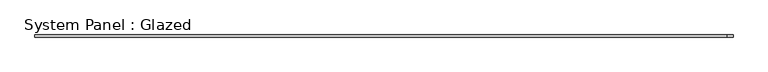
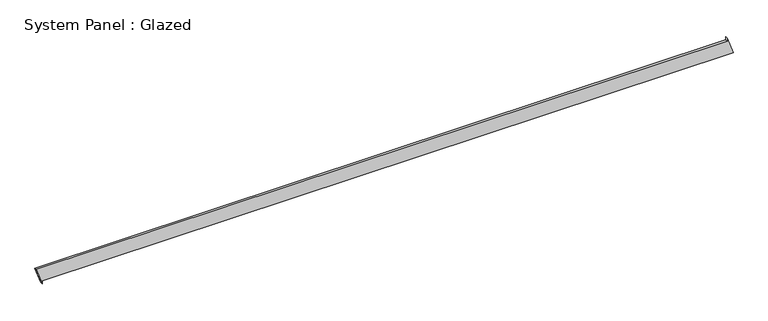
"""IFC4 building model written with IfcOpenShell, lengths in millimetres: plate geometry, System Panel : Glazed."""

import ifcopenshell
import ifcopenshell.guid

model = None  # the IFC model being written
_history = None  # IfcOwnerHistory: only IFC2X3 demands one
_inside = {}  # id of a spatial element -> (the spatial element, [elements in it])
_under = {}  # id of a project, library or spatial element -> (it, [spatial elements below it])
_declared = {}  # id of a project -> (the project, [libraries it declares])
_typed = {}  # id of a type object -> (the type object, [elements of that type])
_made_of = {}  # id of a material, layer set ... -> (it, [elements and type objects made of it])


def new_model(schema):
    """Start an empty IFC model of exactly this schema.

    Asked for "IFC4X3", IfcOpenShell would pick the latest addendum, in which some entities
    have other attributes; the version numbers below select the first issue.
    IFC2X3 requires an IfcOwnerHistory on every rooted entity: one is made here for all.
    """
    global model, _history
    if schema == "IFC4X3":
        model = ifcopenshell.file(schema_version=(4, 3, 0, 0))
    else:
        model = ifcopenshell.file(schema=schema)
    _inside.clear()
    _under.clear()
    _declared.clear()
    _typed.clear()
    _made_of.clear()
    _history = None
    if model.schema == "IFC2X3":
        org = make("IfcOrganization", Name="unknown")
        user = make(
            "IfcPersonAndOrganization",
            ThePerson=make("IfcPerson", FamilyName="unknown"),
            TheOrganization=org,
        )
        app = make(
            "IfcApplication",
            ApplicationDeveloper=org,
            Version="unknown",
            ApplicationFullName="unknown",
            ApplicationIdentifier="unknown",
        )
        _history = make(
            "IfcOwnerHistory",
            OwningUser=user,
            OwningApplication=app,
            ChangeAction="ADDED",
            CreationDate=0,
        )
    return model


def make(cls, **values):
    """One entity of the class cls with the attributes given. An attribute that is None is left unset."""
    return model.create_entity(
        cls, **{name: value for name, value in values.items() if value is not None}
    )


def rooted(cls, **values):
    """An entity with a GlobalId (a new one), such as an element, a storey or a relation."""
    return make(cls, GlobalId=ifcopenshell.guid.new(), OwnerHistory=_history, **values)


def si_unit(unit_type, name, prefix=None):
    """IfcSIUnit, for example si_unit("LENGTHUNIT", "METRE", prefix="MILLI")."""
    return make("IfcSIUnit", UnitType=unit_type, Prefix=prefix, Name=name)


def assignment(units):
    """IfcUnitAssignment: the units of a project."""
    return None if units is None else make("IfcUnitAssignment", Units=units)


def point(xyz):
    """IfcCartesianPoint."""
    return None if xyz is None else make("IfcCartesianPoint", Coordinates=xyz)


def direction(xyz):
    """IfcDirection."""
    return None if xyz is None else make("IfcDirection", DirectionRatios=xyz)


def frame(location, z_axis=None, x_axis=None):
    """IfcAxis2Placement3D, a coordinate frame: its origin and axes. An axis left out is left unset."""
    return make(
        "IfcAxis2Placement3D",
        Location=point(location),
        Axis=direction(z_axis),
        RefDirection=direction(x_axis),
    )


def origin():
    """The frame at (0, 0, 0) with its axes left unset."""
    return frame((0.0, 0.0, 0.0))


def place(relative_to, where):
    """IfcLocalPlacement: puts the frame where relative to a parent placement (None: the world)."""
    return make(
        "IfcLocalPlacement", PlacementRelTo=relative_to, RelativePlacement=where
    )


def context(
    kind, dimensions, precision=None, world=None, true_north=None, identifier=None
):
    """IfcGeometricRepresentationContext, for example the 3D "Model" context."""
    return make(
        "IfcGeometricRepresentationContext",
        ContextIdentifier=identifier,
        ContextType=kind,
        CoordinateSpaceDimension=dimensions,
        Precision=precision,
        WorldCoordinateSystem=world,
        TrueNorth=true_north,
    )


def project(units=None, contexts=None):
    """IfcProject with its units and contexts."""
    return rooted(
        "IfcProject",
        Name="project",
        RepresentationContexts=contexts,
        UnitsInContext=assignment(units),
    )


def spatial(cls, under=None, at=None, **own):
    """A site, building, storey or space (cls), placed at a placement, below another one or the project."""
    s = rooted(cls, ObjectPlacement=at, **own)
    if under is not None:
        _under.setdefault(under.id(), (under, []))[1].append(s)
    return s


def polyline(points):
    """IfcPolyline through the points."""
    return make("IfcPolyline", Points=[point(p) for p in points])


def outline(outer, holes=None, kind="AREA"):
    """IfcArbitraryClosedProfileDef: a profile drawn as a closed curve; with holes, ...WithVoids."""
    if holes is None:
        return make("IfcArbitraryClosedProfileDef", ProfileType=kind, OuterCurve=outer)
    return make(
        "IfcArbitraryProfileDefWithVoids",
        ProfileType=kind,
        OuterCurve=outer,
        InnerCurves=holes,
    )


def extrude(swept, where, along, depth):
    """IfcExtrudedAreaSolid: the profile swept, set in the frame where, extruded along a direction by depth."""
    return make(
        "IfcExtrudedAreaSolid",
        SweptArea=swept,
        Position=where,
        ExtrudedDirection=direction(along),
        Depth=depth,
    )


def shape(context_of_items, identifier, shape_type, items):
    """IfcShapeRepresentation: the items that make up one representation, for example the "Body"."""
    return make(
        "IfcShapeRepresentation",
        ContextOfItems=context_of_items,
        RepresentationIdentifier=identifier,
        RepresentationType=shape_type,
        Items=items,
    )


def source(mapping_origin, context_of_items, identifier, shape_type, items):
    """IfcRepresentationMap: a shape defined once, which mapped items show again and again."""
    return make(
        "IfcRepresentationMap",
        MappingOrigin=mapping_origin,
        MappedRepresentation=shape(context_of_items, identifier, shape_type, items),
    )


def transform(
    local_origin,
    x_axis=None,
    y_axis=None,
    z_axis=None,
    scale=None,
    scale2=None,
    scale3=None,
    uniform=True,
):
    """IfcCartesianTransformationOperator3D, or its non-uniform kind. x_axis, y_axis, z_axis: its Axis1, 2, 3."""
    if uniform:
        return make(
            "IfcCartesianTransformationOperator3D",
            Axis1=direction(x_axis),
            Axis2=direction(y_axis),
            LocalOrigin=point(local_origin),
            Scale=scale,
            Axis3=direction(z_axis),
        )
    return make(
        "IfcCartesianTransformationOperator3DnonUniform",
        Axis1=direction(x_axis),
        Axis2=direction(y_axis),
        LocalOrigin=point(local_origin),
        Scale=scale,
        Axis3=direction(z_axis),
        Scale2=scale2,
        Scale3=scale3,
    )


def mapped(mapping_source, mapping_target):
    """IfcMappedItem: shows the shape of a source again, moved by a transform."""
    return make(
        "IfcMappedItem", MappingSource=mapping_source, MappingTarget=mapping_target
    )


def made_of(thing, what):
    """Note that an element or type object is made of a material, layer set ...; save() writes the relation."""
    if what is not None:
        _made_of.setdefault(what.id(), (what, []))[1].append(thing)
    return thing


def element(
    cls,
    number,
    at=None,
    inside=None,
    cuts=None,
    type_object=None,
    material=None,
    context=None,
    identifier="Body",
    shape_type=None,
    held_by="IfcProductDefinitionShape",
    body=None,
    shapes=None,
    **own,
):
    """One element of the class cls, such as IfcWall. Its Tag is "e" and its number.

    at: its placement. inside: the storey or other place that contains it. cuts: it is an
    opening in that element (IfcRelVoidsElement). A single representation is given by context,
    identifier, shape_type and body (its items); several are given by shapes. held_by: the class
    of the entity that holds the representations. save() writes the other relations.
    """
    e = rooted(cls, Tag="e%d" % number, ObjectPlacement=at, **own)
    if body is not None:
        shapes = [shape(context, identifier, shape_type, body)]
    if shapes is not None:
        e.Representation = make(held_by, Representations=shapes)
    if inside is not None:
        _inside.setdefault(inside.id(), (inside, []))[1].append(e)
    if cuts is not None:
        rooted(
            "IfcRelVoidsElement", RelatingBuildingElement=cuts, RelatedOpeningElement=e
        )
    if type_object is not None:
        _typed.setdefault(type_object.id(), (type_object, []))[1].append(e)
    return made_of(e, material)


def aggregate(whole, parts):
    """IfcRelAggregates: a whole, such as a stair, and the parts it consists of."""
    return rooted("IfcRelAggregates", RelatingObject=whole, RelatedObjects=parts)


def save(model, path):
    """Write the relations noted so far, then the file.

    IfcRelAggregates (storeys below a building ...), IfcRelContainedInSpatialStructure (elements
    in a storey), IfcRelDefinesByType, IfcRelAssociatesMaterial and IfcRelDeclares: one each for
    every whole, place, type object, material and project.
    """
    for whole, parts in _under.values():
        aggregate(whole, parts)
    for where, things in _inside.values():
        rooted(
            "IfcRelContainedInSpatialStructure",
            RelatedElements=things,
            RelatingStructure=where,
        )
    for kind, things in _typed.values():
        rooted("IfcRelDefinesByType", RelatedObjects=things, RelatingType=kind)
    for what, things in _made_of.values():
        rooted("IfcRelAssociatesMaterial", RelatedObjects=things, RelatingMaterial=what)
    for by, libraries in _declared.values():
        rooted("IfcRelDeclares", RelatingContext=by, RelatedDefinitions=libraries)
    model.write(path)


def system_panel_glazed_6fd4334b(model_context):
    return source(origin(), model_context, "Body", "SweptSolid", [
        extrude(outline(polyline([(0.0, -3956.9205184), (35.3553391, -3956.9205184), (35.3553391, 4027.0701191), (235.2094887, 3957.0820623), (199.8541496, 3957.0823635), (199.7861186, -4027.0701191), (0.0, -3956.9205184)])), frame((0.0, -49.5, 0.0), z_axis=(0.0, 1.0, 0.0), x_axis=(0.0, 0.0, 1.0)), (0.0, 0.0, 1.0), 25.0),
    ])


if __name__ == "__main__":
    model = new_model("IFC4")
    model_context = context("Model", 3, world=origin())
    ifc_project = project(units=[si_unit("LENGTHUNIT", "METRE", prefix="MILLI")], contexts=[model_context])
    site = spatial("IfcSite", under=ifc_project)
    building = spatial("IfcBuilding", under=site)
    placement = place(None, origin())
    system_panel_glazed_shape = system_panel_glazed_6fd4334b(model_context)
    element("IfcPlate", 1, ObjectType="System Panel : Glazed", at=placement, inside=building, context=model_context, shape_type="MappedRepresentation", body=[
        mapped(system_panel_glazed_shape, transform((0.0, 0.0, 0.0), x_axis=(1.0, 0.0, 0.0), y_axis=(0.0, 1.0, 0.0), z_axis=(0.0, 0.0, 1.0))),
    ])
    save(model, "model.ifc")

# Revit data of these elements
# Element 1 (IfcPlate, "System Panel : Glazed")
#   Materials on its faces: "Glass"
# Materials
#   "Glass": class "Glass", colour RGB 218 227 224, transparency 0.85, Description = "Soda Lime Glass", Cost = 0
